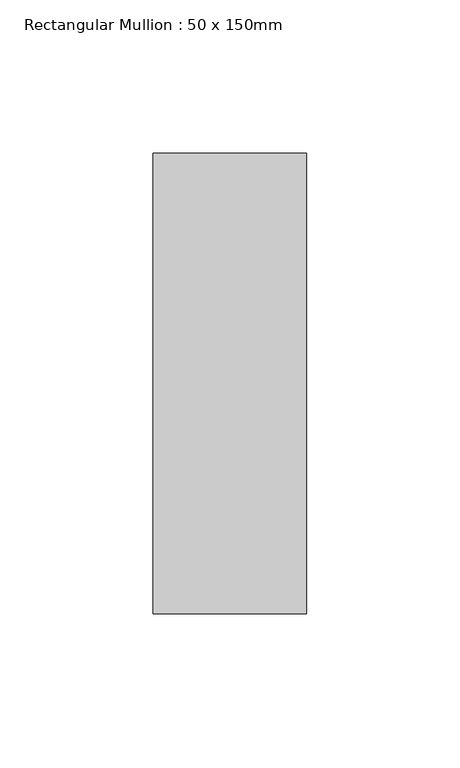
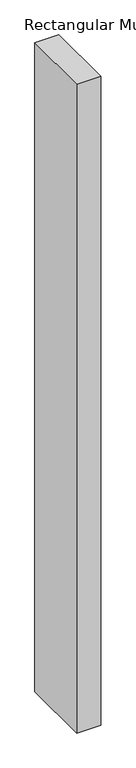
"""IFC4 building model written with IfcOpenShell, lengths in millimetres: member geometry, Rectangular Mullion : 50 x 150mm."""

from ifc_helpers import new_model, si_unit, frame, origin, place, context, project, spatial, polyline, outline, extrude, source, transform, mapped, element, save


def rectangular_mullion_50_x_150mm_379ba6c0(model_context):
    return source(origin(), model_context, "Body", "SweptSolid", [
        extrude(outline(polyline([(0.0, 75.0), (0.0, -75.0), (-50.0, -75.0), (-50.0, 75.0), (0.0, 75.0)])), frame((0.0, 0.0, -1425.0000001), z_axis=(0.0, 0.0, 1.0), x_axis=(1.0, 0.0, 0.0)), (0.0, 0.0, 1.0), 1425.0000001),
    ])


if __name__ == "__main__":
    model = new_model("IFC4")
    model_context = context("Model", 3, world=origin())
    ifc_project = project(units=[si_unit("LENGTHUNIT", "METRE", prefix="MILLI")], contexts=[model_context])
    site = spatial("IfcSite", under=ifc_project)
    building = spatial("IfcBuilding", under=site)
    placement = place(None, origin())
    rectangular_mullion_50_x_150mm_shape = rectangular_mullion_50_x_150mm_379ba6c0(model_context)
    element("IfcMember", 1, ObjectType="Rectangular Mullion : 50 x 150mm", at=placement, inside=building, context=model_context, shape_type="MappedRepresentation", body=[
        mapped(rectangular_mullion_50_x_150mm_shape, transform((0.0, 0.0, 0.0), x_axis=(1.0, 0.0, 0.0), y_axis=(0.0, 1.0, 0.0), z_axis=(0.0, 0.0, 1.0))),
    ])
    save(model, "model.ifc")

# Revit data of these elements
# Type "Rectangular Mullion : 50 x 150mm"
#   built-in parameter 1007304 = 0.492126 (stored number, unit not read)
#   built-in parameter 1007301 = 0.082021 (stored number, unit not read)
#   built-in parameter 1007300 = 0.082021 (stored number, unit not read)
# Element 1 (IfcMember, "Rectangular Mullion : 50 x 150mm")
#   Materials on its faces: "Aluminium"
# Materials
#   "Aluminium": class "Metal", colour RGB 247 247 247, transparency 0, Description = "Aluminium 6061", Cost = 0
